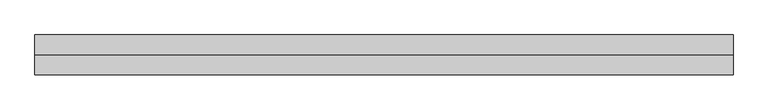
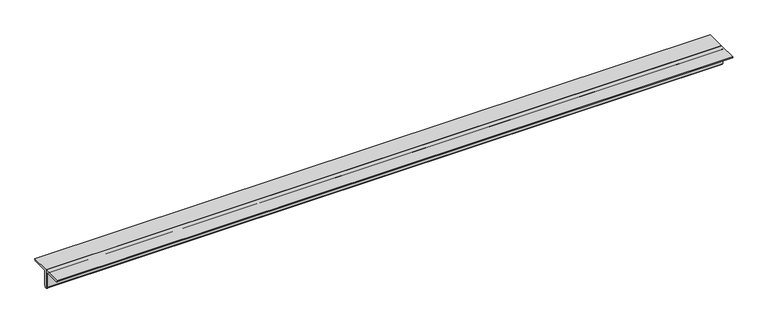
"""IFC4 building model written with IfcOpenShell, lengths in millimetres: member geometry, 0123_Steel Framing_2Ls-KSD3502 : H_SB_AR_S04_2Ls-130x130x12_VBR1."""

import ifcopenshell
import ifcopenshell.guid

model = None  # the IFC model being written
_history = None  # IfcOwnerHistory: only IFC2X3 demands one
_inside = {}  # id of a spatial element -> (the spatial element, [elements in it])
_under = {}  # id of a project, library or spatial element -> (it, [spatial elements below it])
_declared = {}  # id of a project -> (the project, [libraries it declares])
_typed = {}  # id of a type object -> (the type object, [elements of that type])
_made_of = {}  # id of a material, layer set ... -> (it, [elements and type objects made of it])


def new_model(schema):
    """Start an empty IFC model of exactly this schema.

    Asked for "IFC4X3", IfcOpenShell would pick the latest addendum, in which some entities
    have other attributes; the version numbers below select the first issue.
    IFC2X3 requires an IfcOwnerHistory on every rooted entity: one is made here for all.
    """
    global model, _history
    if schema == "IFC4X3":
        model = ifcopenshell.file(schema_version=(4, 3, 0, 0))
    else:
        model = ifcopenshell.file(schema=schema)
    _inside.clear()
    _under.clear()
    _declared.clear()
    _typed.clear()
    _made_of.clear()
    _history = None
    if model.schema == "IFC2X3":
        org = make("IfcOrganization", Name="unknown")
        user = make(
            "IfcPersonAndOrganization",
            ThePerson=make("IfcPerson", FamilyName="unknown"),
            TheOrganization=org,
        )
        app = make(
            "IfcApplication",
            ApplicationDeveloper=org,
            Version="unknown",
            ApplicationFullName="unknown",
            ApplicationIdentifier="unknown",
        )
        _history = make(
            "IfcOwnerHistory",
            OwningUser=user,
            OwningApplication=app,
            ChangeAction="ADDED",
            CreationDate=0,
        )
    return model


def make(cls, **values):
    """One entity of the class cls with the attributes given. An attribute that is None is left unset."""
    return model.create_entity(
        cls, **{name: value for name, value in values.items() if value is not None}
    )


def rooted(cls, **values):
    """An entity with a GlobalId (a new one), such as an element, a storey or a relation."""
    return make(cls, GlobalId=ifcopenshell.guid.new(), OwnerHistory=_history, **values)


def si_unit(unit_type, name, prefix=None):
    """IfcSIUnit, for example si_unit("LENGTHUNIT", "METRE", prefix="MILLI")."""
    return make("IfcSIUnit", UnitType=unit_type, Prefix=prefix, Name=name)


def assignment(units):
    """IfcUnitAssignment: the units of a project."""
    return None if units is None else make("IfcUnitAssignment", Units=units)


def point(xyz):
    """IfcCartesianPoint."""
    return None if xyz is None else make("IfcCartesianPoint", Coordinates=xyz)


def direction(xyz):
    """IfcDirection."""
    return None if xyz is None else make("IfcDirection", DirectionRatios=xyz)


def frame(location, z_axis=None, x_axis=None):
    """IfcAxis2Placement3D, a coordinate frame: its origin and axes. An axis left out is left unset."""
    return make(
        "IfcAxis2Placement3D",
        Location=point(location),
        Axis=direction(z_axis),
        RefDirection=direction(x_axis),
    )


def frame_2d(location, x_axis=None):
    """IfcAxis2Placement2D, a coordinate frame in the plane: its origin and x axis."""
    return make(
        "IfcAxis2Placement2D", Location=point(location), RefDirection=direction(x_axis)
    )


def origin():
    """The frame at (0, 0, 0) with its axes left unset."""
    return frame((0.0, 0.0, 0.0))


def place(relative_to, where):
    """IfcLocalPlacement: puts the frame where relative to a parent placement (None: the world)."""
    return make(
        "IfcLocalPlacement", PlacementRelTo=relative_to, RelativePlacement=where
    )


def context(
    kind, dimensions, precision=None, world=None, true_north=None, identifier=None
):
    """IfcGeometricRepresentationContext, for example the 3D "Model" context."""
    return make(
        "IfcGeometricRepresentationContext",
        ContextIdentifier=identifier,
        ContextType=kind,
        CoordinateSpaceDimension=dimensions,
        Precision=precision,
        WorldCoordinateSystem=world,
        TrueNorth=true_north,
    )


def project(units=None, contexts=None):
    """IfcProject with its units and contexts."""
    return rooted(
        "IfcProject",
        Name="project",
        RepresentationContexts=contexts,
        UnitsInContext=assignment(units),
    )


def spatial(cls, under=None, at=None, **own):
    """A site, building, storey or space (cls), placed at a placement, below another one or the project."""
    s = rooted(cls, ObjectPlacement=at, **own)
    if under is not None:
        _under.setdefault(under.id(), (under, []))[1].append(s)
    return s


def polyline(points):
    """IfcPolyline through the points."""
    return make("IfcPolyline", Points=[point(p) for p in points])


def circle_curve(where, radius):
    """IfcCircle in the frame where."""
    return make("IfcCircle", Position=where, Radius=radius)


def trimmed(basis, trim1, trim2, sense, master):
    """IfcTrimmedCurve: the piece of a basis curve between two trims."""
    return make(
        "IfcTrimmedCurve",
        BasisCurve=basis,
        Trim1=trim1,
        Trim2=trim2,
        SenseAgreement=sense,
        MasterRepresentation=master,
    )


def segment(curve, same_sense, transition):
    """IfcCompositeCurveSegment."""
    return make(
        "IfcCompositeCurveSegment",
        Transition=transition,
        SameSense=same_sense,
        ParentCurve=curve,
    )


def composite_curve(segments, self_intersect=None):
    """IfcCompositeCurve: segments joined end to end."""
    return make("IfcCompositeCurve", Segments=segments, SelfIntersect=self_intersect)


def outline(outer, holes=None, kind="AREA"):
    """IfcArbitraryClosedProfileDef: a profile drawn as a closed curve; with holes, ...WithVoids."""
    if holes is None:
        return make("IfcArbitraryClosedProfileDef", ProfileType=kind, OuterCurve=outer)
    return make(
        "IfcArbitraryProfileDefWithVoids",
        ProfileType=kind,
        OuterCurve=outer,
        InnerCurves=holes,
    )


def extrude(swept, where, along, depth):
    """IfcExtrudedAreaSolid: the profile swept, set in the frame where, extruded along a direction by depth."""
    return make(
        "IfcExtrudedAreaSolid",
        SweptArea=swept,
        Position=where,
        ExtrudedDirection=direction(along),
        Depth=depth,
    )


def shape(context_of_items, identifier, shape_type, items):
    """IfcShapeRepresentation: the items that make up one representation, for example the "Body"."""
    return make(
        "IfcShapeRepresentation",
        ContextOfItems=context_of_items,
        RepresentationIdentifier=identifier,
        RepresentationType=shape_type,
        Items=items,
    )


def source(mapping_origin, context_of_items, identifier, shape_type, items):
    """IfcRepresentationMap: a shape defined once, which mapped items show again and again."""
    return make(
        "IfcRepresentationMap",
        MappingOrigin=mapping_origin,
        MappedRepresentation=shape(context_of_items, identifier, shape_type, items),
    )


def transform(
    local_origin,
    x_axis=None,
    y_axis=None,
    z_axis=None,
    scale=None,
    scale2=None,
    scale3=None,
    uniform=True,
):
    """IfcCartesianTransformationOperator3D, or its non-uniform kind. x_axis, y_axis, z_axis: its Axis1, 2, 3."""
    if uniform:
        return make(
            "IfcCartesianTransformationOperator3D",
            Axis1=direction(x_axis),
            Axis2=direction(y_axis),
            LocalOrigin=point(local_origin),
            Scale=scale,
            Axis3=direction(z_axis),
        )
    return make(
        "IfcCartesianTransformationOperator3DnonUniform",
        Axis1=direction(x_axis),
        Axis2=direction(y_axis),
        LocalOrigin=point(local_origin),
        Scale=scale,
        Axis3=direction(z_axis),
        Scale2=scale2,
        Scale3=scale3,
    )


def mapped(mapping_source, mapping_target):
    """IfcMappedItem: shows the shape of a source again, moved by a transform."""
    return make(
        "IfcMappedItem", MappingSource=mapping_source, MappingTarget=mapping_target
    )


def made_of(thing, what):
    """Note that an element or type object is made of a material, layer set ...; save() writes the relation."""
    if what is not None:
        _made_of.setdefault(what.id(), (what, []))[1].append(thing)
    return thing


def element(
    cls,
    number,
    at=None,
    inside=None,
    cuts=None,
    type_object=None,
    material=None,
    context=None,
    identifier="Body",
    shape_type=None,
    held_by="IfcProductDefinitionShape",
    body=None,
    shapes=None,
    **own,
):
    """One element of the class cls, such as IfcWall. Its Tag is "e" and its number.

    at: its placement. inside: the storey or other place that contains it. cuts: it is an
    opening in that element (IfcRelVoidsElement). A single representation is given by context,
    identifier, shape_type and body (its items); several are given by shapes. held_by: the class
    of the entity that holds the representations. save() writes the other relations.
    """
    e = rooted(cls, Tag="e%d" % number, ObjectPlacement=at, **own)
    if body is not None:
        shapes = [shape(context, identifier, shape_type, body)]
    if shapes is not None:
        e.Representation = make(held_by, Representations=shapes)
    if inside is not None:
        _inside.setdefault(inside.id(), (inside, []))[1].append(e)
    if cuts is not None:
        rooted(
            "IfcRelVoidsElement", RelatingBuildingElement=cuts, RelatedOpeningElement=e
        )
    if type_object is not None:
        _typed.setdefault(type_object.id(), (type_object, []))[1].append(e)
    return made_of(e, material)


def aggregate(whole, parts):
    """IfcRelAggregates: a whole, such as a stair, and the parts it consists of."""
    return rooted("IfcRelAggregates", RelatingObject=whole, RelatedObjects=parts)


def save(model, path):
    """Write the relations noted so far, then the file.

    IfcRelAggregates (storeys below a building ...), IfcRelContainedInSpatialStructure (elements
    in a storey), IfcRelDefinesByType, IfcRelAssociatesMaterial and IfcRelDeclares: one each for
    every whole, place, type object, material and project.
    """
    for whole, parts in _under.values():
        aggregate(whole, parts)
    for where, things in _inside.values():
        rooted(
            "IfcRelContainedInSpatialStructure",
            RelatedElements=things,
            RelatingStructure=where,
        )
    for kind, things in _typed.values():
        rooted("IfcRelDefinesByType", RelatedObjects=things, RelatingType=kind)
    for what, things in _made_of.values():
        rooted("IfcRelAssociatesMaterial", RelatedObjects=things, RelatingMaterial=what)
    for by, libraries in _declared.values():
        rooted("IfcRelDeclares", RelatingContext=by, RelatedDefinitions=libraries)
    model.write(path)


def member_5add8e11(model_context):
    return source(origin(), model_context, "Body", "SweptSolid", [
        extrude(outline(composite_curve([segment(polyline([(0.0, 36.4), (130.0, 36.4)]), True, "CONTINUOUS"), segment(trimmed(circle_curve(frame_2d((118.0, 36.4)), 12.0), [point((130.0, 36.4))], [point((118.0, 24.4))], False, "CARTESIAN"), True, "CONTINUOUS"), segment(polyline([(118.0, 24.4), (24.0, 24.4)]), True, "CONTINUOUS"), segment(trimmed(circle_curve(frame_2d((24.0, 12.4)), 12.0), [point((24.0, 24.4))], [point((12.0, 12.4))], True, "CARTESIAN"), True, "CONTINUOUS"), segment(polyline([(12.0, 12.4), (12.0, -81.6)]), True, "CONTINUOUS"), segment(trimmed(circle_curve(frame_2d((0.0, -81.6)), 12.0), [point((12.0, -81.6))], [point((0.0, -93.6))], False, "CARTESIAN"), True, "CONTINUOUS"), segment(polyline([(0.0, -93.6), (0.0, 36.4)]), True, "CONTINUOUS")], self_intersect=False)), frame((-2281.9000111, 0.0, 0.0), z_axis=(1.0, 0.0, 0.0), x_axis=(0.0, 1.0, 0.0)), (0.0, 0.0, 1.0), 4563.8000221),
        extrude(outline(composite_curve([segment(polyline([(0.0, 36.4), (0.0, -93.6)]), True, "CONTINUOUS"), segment(trimmed(circle_curve(frame_2d((0.0, -81.6)), 12.0), [point((0.0, -93.6))], [point((-12.0, -81.6))], False, "CARTESIAN"), True, "CONTINUOUS"), segment(polyline([(-12.0, -81.6), (-12.0, 12.4)]), True, "CONTINUOUS"), segment(trimmed(circle_curve(frame_2d((-24.0, 12.4)), 12.0), [point((-12.0, 12.4))], [point((-24.0, 24.4))], True, "CARTESIAN"), True, "CONTINUOUS"), segment(polyline([(-24.0, 24.4), (-118.0, 24.4)]), True, "CONTINUOUS"), segment(trimmed(circle_curve(frame_2d((-118.0, 36.4)), 12.0), [point((-118.0, 24.4))], [point((-130.0, 36.4))], False, "CARTESIAN"), True, "CONTINUOUS"), segment(polyline([(-130.0, 36.4), (0.0, 36.4)]), True, "CONTINUOUS")], self_intersect=False)), frame((-2281.9000111, 0.0, 0.0), z_axis=(1.0, 0.0, 0.0), x_axis=(0.0, 1.0, 0.0)), (0.0, 0.0, 1.0), 4563.8000221),
    ])


if __name__ == "__main__":
    model = new_model("IFC4")
    model_context = context("Model", 3, world=origin())
    ifc_project = project(units=[si_unit("LENGTHUNIT", "METRE", prefix="MILLI")], contexts=[model_context])
    site = spatial("IfcSite", under=ifc_project)
    building = spatial("IfcBuilding", under=site)
    placement = place(None, origin())
    member_shape = member_5add8e11(model_context)
    element("IfcMember", 1, ObjectType="0123_Steel Framing_2Ls-KSD3502 : H_SB_AR_S04_2Ls-130x130x12_VBR1", at=placement, inside=building, context=model_context, shape_type="MappedRepresentation", body=[
        mapped(member_shape, transform((0.0, 0.0, 0.0), x_axis=(1.0, 0.0, 0.0), y_axis=(0.0, 1.0, 0.0), z_axis=(0.0, 0.0, 1.0))),
    ])
    save(model, "model.ifc")

# Revit data of these elements
# Type "0123_Steel Framing_2Ls-KSD3502 : H_SB_AR_S04_2Ls-130x130x12_VBR1"
#   Assembly Code = "B10"
#   Legs = "SLBB"
#   W = 8.97
#   Perimeter = 1.04 m²/m
#   Nominal Weight = 46.80 kgf/m
#   Length [instance default] = 1000 mm
#   Space = 0 mm
#   b = 130 mm
#   d = 130 mm
#   t = 12 mm
#   y = 36.4 mm
#   A = 0.005952 m²
#   Structural Material [instance default] = Steel ASTM A36
# Element 1 (IfcMember, "0123_Steel Framing_2Ls-KSD3502 : H_SB_AR_S04_2Ls-130x130x12_VBR1")
#   Structural Material = Steel, 45-345
#   Materials on its faces: "Steel, 45-345"
# Materials
#   "Steel ASTM A36": class "Metal", colour RGB 199 199 199, transparency 0, Description = "Structural steel, ASTM A36 Grade B, mill finish", Cost = 0
#   "Steel, 45-345": class "Metal", colour RGB 189 187 185, transparency 0, Description = "Steel 345 MPa", Cost = 0
